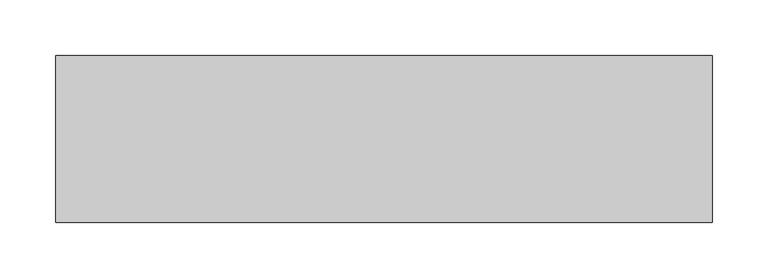
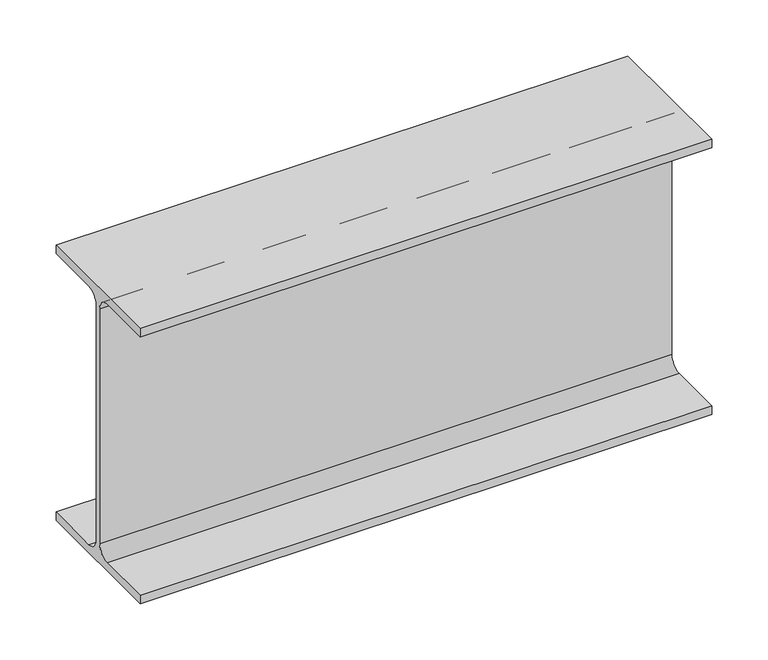
"""IFC4 building model written with IfcOpenShell, lengths in millimetres: beam geometry, 0912_Steel Framing_H-KSD3502 : H_SB_ASB_H-300x150x6.5x9."""

from ifc_helpers import new_model, si_unit, point, frame, frame_2d, origin, place, context, project, spatial, polyline, circle_curve, trimmed, segment, composite_curve, outline, extrude, source, transform, mapped, element, save


def beam_8e0ea4b8(model_context):
    return source(origin(), model_context, "Body", "SweptSolid", [
        extrude(outline(composite_curve([segment(polyline([(-75.0, -141.0), (-16.25, -141.0)]), True, "CONTINUOUS"), segment(trimmed(circle_curve(frame_2d((-16.25, -128.0)), 13.0), [point((-16.25, -141.0))], [point((-3.25, -128.0))], True, "CARTESIAN"), True, "CONTINUOUS"), segment(polyline([(-3.25, -128.0), (-3.25, 128.0)]), True, "CONTINUOUS"), segment(trimmed(circle_curve(frame_2d((-16.25, 128.0)), 13.0), [point((-3.25, 128.0))], [point((-16.25, 141.0))], True, "CARTESIAN"), True, "CONTINUOUS"), segment(polyline([(-16.25, 141.0), (-75.0, 141.0), (-75.0, 150.0), (75.0, 150.0), (75.0, 141.0), (16.25, 141.0)]), True, "CONTINUOUS"), segment(trimmed(circle_curve(frame_2d((16.25, 128.0)), 13.0), [point((16.25, 141.0))], [point((3.25, 128.0))], True, "CARTESIAN"), True, "CONTINUOUS"), segment(polyline([(3.25, 128.0), (3.25, -128.0)]), True, "CONTINUOUS"), segment(trimmed(circle_curve(frame_2d((16.25, -128.0)), 13.0), [point((3.25, -128.0))], [point((16.25, -141.0))], True, "CARTESIAN"), True, "CONTINUOUS"), segment(polyline([(16.25, -141.0), (75.0, -141.0), (75.0, -150.0), (-75.0, -150.0), (-75.0, -141.0)]), True, "CONTINUOUS")], self_intersect=False)), frame((-282.3, 0.0, 0.0), z_axis=(1.0, 0.0, 0.0), x_axis=(0.0, 1.0, 0.0)), (0.0, 0.0, 1.0), 589.6),
    ])


if __name__ == "__main__":
    model = new_model("IFC4")
    model_context = context("Model", 3, world=origin())
    ifc_project = project(units=[si_unit("LENGTHUNIT", "METRE", prefix="MILLI")], contexts=[model_context])
    site = spatial("IfcSite", under=ifc_project)
    building = spatial("IfcBuilding", under=site)
    placement = place(None, origin())
    beam_shape = beam_8e0ea4b8(model_context)
    element("IfcBeam", 1, ObjectType="0912_Steel Framing_H-KSD3502 : H_SB_ASB_H-300x150x6.5x9", at=placement, inside=building, context=model_context, shape_type="MappedRepresentation", body=[
        mapped(beam_shape, transform((0.0, 0.0, 0.0), x_axis=(1.0, 0.0, 0.0), y_axis=(0.0, 1.0, 0.0), z_axis=(0.0, 0.0, 1.0))),
    ])
    save(model, "model.ifc")

# Revit data of these elements
# Type "0912_Steel Framing_H-KSD3502 : H_SB_ASB_H-300x150x6.5x9"
#   H_WM Code_1 = "S01AA002-00001 | Main Steel Structure Fabrication Work | Shelter/Building | Medium Steel - Standard (90KG/M>Weight≥30KG/M) | Material: (   )"
#   H_WM Code_2 = "S03AA028-00001 | Main Steel Structure Erection Work | Shelter/Building | Medium Steel (90KG/M>Weight≥30KG/M) | Material: (   )"
#   H_WM Code_3 = "S01AA010-00001 | Main Steel Structure Fabrication Work | Shelter/Building | Steel Painting/Coating | for Non-Fireproofed Steel Surface, Surface Preparation, Primer, Second & Final Coat | Material: (   )"
#   H_Q'ty Cal Type Tag = "SB-Q2"
#   Width = 15.0 cm
#   Web Thickness = 0.65 cm
#   Web Fillet = 1.3 cm
#   Warping Constant = 107000.0 cm⁶
#   W = 0
#   Torsional Moment of Inertia = 9.9539 cm⁴
#   Section Area = 46.78 cm²
#   Plastic Modulus weak axis = 105.0 cm³
#   Plastic Modulus strong axis = 542.0 cm³
#   Perimeter = 1.17 m²/m
#   Nominal Weight = 36.70 kgf/m
#   Moment of Inertia weak axis = 508.00 cm⁴
#   Moment of Inertia strong axis = 7210.00 cm⁴
#   Height = 30.0 cm
#   Flange Thickness = 0.9 cm
#   Elastic Modulus weak axis = 67.7 cm³
#   Elastic Modulus strong axis = 481.0 cm³
#   Centroid Vertical = 15.0 cm
#   Centroid Horizontal = 7.5 cm
#   Ix = 72100000
#   Length [instance default] = 1.5240 m
#   Zx = 542000
#   b = 0.1500 m
#   h = 0.3000 m
#   r = 0.0130 m
#   s = 0.0065 m
#   t = 0.0090 m
#   A = 0.004678 m²
#   Structural Material [instance default] = Steel, 45-345
#   Assembly Code = ""
# Element 1 (IfcBeam, "0912_Steel Framing_H-KSD3502 : H_SB_ASB_H-300x150x6.5x9")
#   Structural Material = none
# Materials
#   "Steel, 45-345": class "Metal", colour RGB 189 187 185, transparency 0, Description = "Steel 345 MPa", Cost = 0
